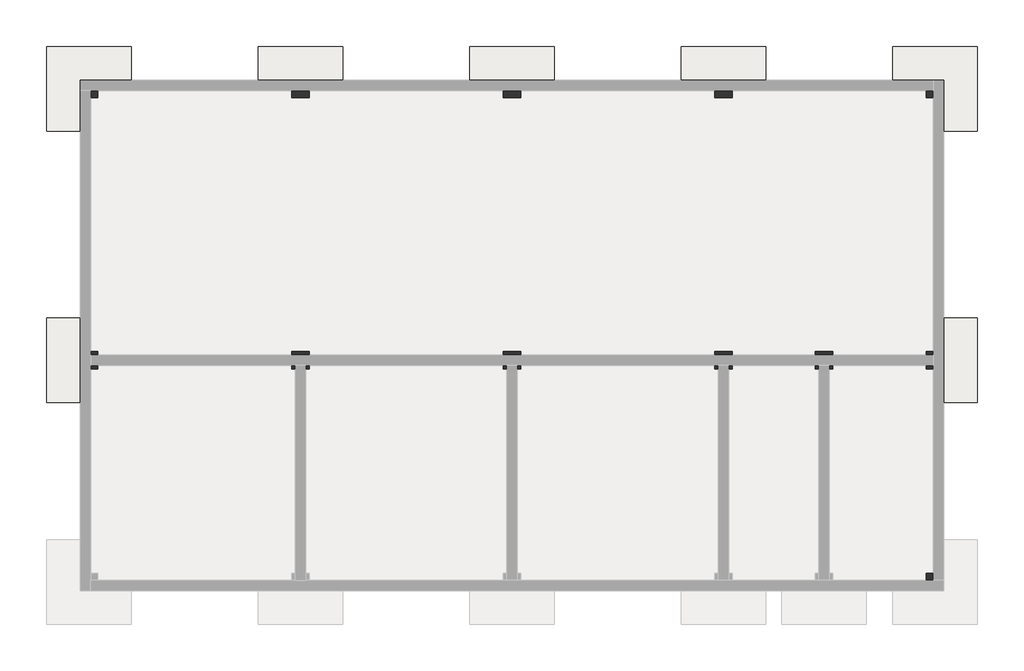
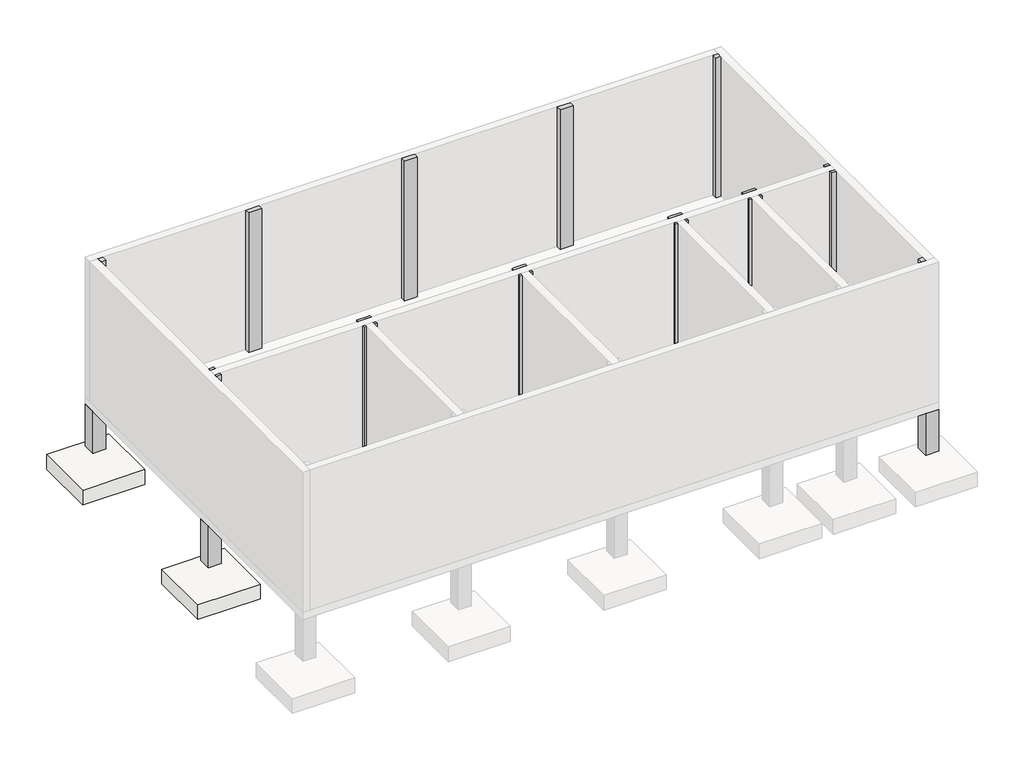
# One storey, part 2 of 2: 24 columns, 11 slabs.
"""IFC4 building model written with IfcOpenShell, lengths in millimetres."""

import ifcopenshell
import ifcopenshell.guid

model = None  # the IFC model being written
_history = None  # IfcOwnerHistory: only IFC2X3 demands one
_inside = {}  # id of a spatial element -> (the spatial element, [elements in it])
_under = {}  # id of a project, library or spatial element -> (it, [spatial elements below it])
_declared = {}  # id of a project -> (the project, [libraries it declares])
_typed = {}  # id of a type object -> (the type object, [elements of that type])
_made_of = {}  # id of a material, layer set ... -> (it, [elements and type objects made of it])


def new_model(schema):
    """Start an empty IFC model of exactly this schema.

    Asked for "IFC4X3", IfcOpenShell would pick the latest addendum, in which some entities
    have other attributes; the version numbers below select the first issue.
    IFC2X3 requires an IfcOwnerHistory on every rooted entity: one is made here for all.
    """
    global model, _history
    if schema == "IFC4X3":
        model = ifcopenshell.file(schema_version=(4, 3, 0, 0))
    else:
        model = ifcopenshell.file(schema=schema)
    _inside.clear()
    _under.clear()
    _declared.clear()
    _typed.clear()
    _made_of.clear()
    _history = None
    if model.schema == "IFC2X3":
        org = make("IfcOrganization", Name="unknown")
        user = make(
            "IfcPersonAndOrganization",
            ThePerson=make("IfcPerson", FamilyName="unknown"),
            TheOrganization=org,
        )
        app = make(
            "IfcApplication",
            ApplicationDeveloper=org,
            Version="unknown",
            ApplicationFullName="unknown",
            ApplicationIdentifier="unknown",
        )
        _history = make(
            "IfcOwnerHistory",
            OwningUser=user,
            OwningApplication=app,
            ChangeAction="ADDED",
            CreationDate=0,
        )
    return model


def make(cls, **values):
    """One entity of the class cls with the attributes given. An attribute that is None is left unset."""
    return model.create_entity(
        cls, **{name: value for name, value in values.items() if value is not None}
    )


def rooted(cls, **values):
    """An entity with a GlobalId (a new one), such as an element, a storey or a relation."""
    return make(cls, GlobalId=ifcopenshell.guid.new(), OwnerHistory=_history, **values)


def si_unit(unit_type, name, prefix=None):
    """IfcSIUnit, for example si_unit("LENGTHUNIT", "METRE", prefix="MILLI")."""
    return make("IfcSIUnit", UnitType=unit_type, Prefix=prefix, Name=name)


def assignment(units):
    """IfcUnitAssignment: the units of a project."""
    return None if units is None else make("IfcUnitAssignment", Units=units)


def point(xyz):
    """IfcCartesianPoint."""
    return None if xyz is None else make("IfcCartesianPoint", Coordinates=xyz)


def direction(xyz):
    """IfcDirection."""
    return None if xyz is None else make("IfcDirection", DirectionRatios=xyz)


def frame(location, z_axis=None, x_axis=None):
    """IfcAxis2Placement3D, a coordinate frame: its origin and axes. An axis left out is left unset."""
    return make(
        "IfcAxis2Placement3D",
        Location=point(location),
        Axis=direction(z_axis),
        RefDirection=direction(x_axis),
    )


def origin():
    """The frame at (0, 0, 0) with its axes left unset."""
    return frame((0.0, 0.0, 0.0))


def place(relative_to, where):
    """IfcLocalPlacement: puts the frame where relative to a parent placement (None: the world)."""
    return make(
        "IfcLocalPlacement", PlacementRelTo=relative_to, RelativePlacement=where
    )


def context(
    kind, dimensions, precision=None, world=None, true_north=None, identifier=None
):
    """IfcGeometricRepresentationContext, for example the 3D "Model" context."""
    return make(
        "IfcGeometricRepresentationContext",
        ContextIdentifier=identifier,
        ContextType=kind,
        CoordinateSpaceDimension=dimensions,
        Precision=precision,
        WorldCoordinateSystem=world,
        TrueNorth=true_north,
    )


def project(units=None, contexts=None):
    """IfcProject with its units and contexts."""
    return rooted(
        "IfcProject",
        Name="project",
        RepresentationContexts=contexts,
        UnitsInContext=assignment(units),
    )


def spatial(cls, under=None, at=None, **own):
    """A site, building, storey or space (cls), placed at a placement, below another one or the project."""
    s = rooted(cls, ObjectPlacement=at, **own)
    if under is not None:
        _under.setdefault(under.id(), (under, []))[1].append(s)
    return s


def polyline(points):
    """IfcPolyline through the points."""
    return make("IfcPolyline", Points=[point(p) for p in points])


def outline(outer, holes=None, kind="AREA"):
    """IfcArbitraryClosedProfileDef: a profile drawn as a closed curve; with holes, ...WithVoids."""
    if holes is None:
        return make("IfcArbitraryClosedProfileDef", ProfileType=kind, OuterCurve=outer)
    return make(
        "IfcArbitraryProfileDefWithVoids",
        ProfileType=kind,
        OuterCurve=outer,
        InnerCurves=holes,
    )


def extrude(swept, where, along, depth):
    """IfcExtrudedAreaSolid: the profile swept, set in the frame where, extruded along a direction by depth."""
    return make(
        "IfcExtrudedAreaSolid",
        SweptArea=swept,
        Position=where,
        ExtrudedDirection=direction(along),
        Depth=depth,
    )


def faces_of(points, faces, orient=None, outer=None):
    """IfcFace entities. A face is a list of loops; a loop is a list of indices into points, from 0.

    orient and outer hold one flag for each loop. By default every Orientation is true, the
    first loop of a face is its IfcFaceOuterBound and the others are IfcFaceBound.
    """
    made = []
    for i, loops in enumerate(faces):
        bounds = []
        for j, loop in enumerate(loops):
            is_outer = j == 0 if outer is None else outer[i][j]
            bounds.append(
                make(
                    "IfcFaceOuterBound" if is_outer else "IfcFaceBound",
                    Bound=make("IfcPolyLoop", Polygon=[points[k] for k in loop]),
                    Orientation=True if orient is None else orient[i][j],
                )
            )
        made.append(make("IfcFace", Bounds=bounds))
    return made


def faceted_brep(points, faces, orient=None, outer=None, voids=None):
    """IfcFacetedBrep: a solid bounded by flat faces; with voids (closed shells), ...WithVoids."""
    shared = [point(p) for p in points]
    hull = make("IfcClosedShell", CfsFaces=faces_of(shared, faces, orient, outer))
    if voids is None:
        return make("IfcFacetedBrep", Outer=hull)
    return make(
        "IfcFacetedBrepWithVoids",
        Outer=hull,
        Voids=[
            make(cls, CfsFaces=faces_of(shared, fs, o, b)) for cls, fs, o, b in voids
        ],
    )


def shape(context_of_items, identifier, shape_type, items):
    """IfcShapeRepresentation: the items that make up one representation, for example the "Body"."""
    return make(
        "IfcShapeRepresentation",
        ContextOfItems=context_of_items,
        RepresentationIdentifier=identifier,
        RepresentationType=shape_type,
        Items=items,
    )


def source(mapping_origin, context_of_items, identifier, shape_type, items):
    """IfcRepresentationMap: a shape defined once, which mapped items show again and again."""
    return make(
        "IfcRepresentationMap",
        MappingOrigin=mapping_origin,
        MappedRepresentation=shape(context_of_items, identifier, shape_type, items),
    )


def transform(
    local_origin,
    x_axis=None,
    y_axis=None,
    z_axis=None,
    scale=None,
    scale2=None,
    scale3=None,
    uniform=True,
):
    """IfcCartesianTransformationOperator3D, or its non-uniform kind. x_axis, y_axis, z_axis: its Axis1, 2, 3."""
    if uniform:
        return make(
            "IfcCartesianTransformationOperator3D",
            Axis1=direction(x_axis),
            Axis2=direction(y_axis),
            LocalOrigin=point(local_origin),
            Scale=scale,
            Axis3=direction(z_axis),
        )
    return make(
        "IfcCartesianTransformationOperator3DnonUniform",
        Axis1=direction(x_axis),
        Axis2=direction(y_axis),
        LocalOrigin=point(local_origin),
        Scale=scale,
        Axis3=direction(z_axis),
        Scale2=scale2,
        Scale3=scale3,
    )


def mapped(mapping_source, mapping_target):
    """IfcMappedItem: shows the shape of a source again, moved by a transform."""
    return make(
        "IfcMappedItem", MappingSource=mapping_source, MappingTarget=mapping_target
    )


def made_of(thing, what):
    """Note that an element or type object is made of a material, layer set ...; save() writes the relation."""
    if what is not None:
        _made_of.setdefault(what.id(), (what, []))[1].append(thing)
    return thing


def element(
    cls,
    number,
    at=None,
    inside=None,
    cuts=None,
    type_object=None,
    material=None,
    context=None,
    identifier="Body",
    shape_type=None,
    held_by="IfcProductDefinitionShape",
    body=None,
    shapes=None,
    **own,
):
    """One element of the class cls, such as IfcWall. Its Tag is "e" and its number.

    at: its placement. inside: the storey or other place that contains it. cuts: it is an
    opening in that element (IfcRelVoidsElement). A single representation is given by context,
    identifier, shape_type and body (its items); several are given by shapes. held_by: the class
    of the entity that holds the representations. save() writes the other relations.
    """
    e = rooted(cls, Tag="e%d" % number, ObjectPlacement=at, **own)
    if body is not None:
        shapes = [shape(context, identifier, shape_type, body)]
    if shapes is not None:
        e.Representation = make(held_by, Representations=shapes)
    if inside is not None:
        _inside.setdefault(inside.id(), (inside, []))[1].append(e)
    if cuts is not None:
        rooted(
            "IfcRelVoidsElement", RelatingBuildingElement=cuts, RelatedOpeningElement=e
        )
    if type_object is not None:
        _typed.setdefault(type_object.id(), (type_object, []))[1].append(e)
    return made_of(e, material)


def aggregate(whole, parts):
    """IfcRelAggregates: a whole, such as a stair, and the parts it consists of."""
    return rooted("IfcRelAggregates", RelatingObject=whole, RelatedObjects=parts)


def save(model, path):
    """Write the relations noted so far, then the file.

    IfcRelAggregates (storeys below a building ...), IfcRelContainedInSpatialStructure (elements
    in a storey), IfcRelDefinesByType, IfcRelAssociatesMaterial and IfcRelDeclares: one each for
    every whole, place, type object, material and project.
    """
    for whole, parts in _under.values():
        aggregate(whole, parts)
    for where, things in _inside.values():
        rooted(
            "IfcRelContainedInSpatialStructure",
            RelatedElements=things,
            RelatingStructure=where,
        )
    for kind, things in _typed.values():
        rooted("IfcRelDefinesByType", RelatedObjects=things, RelatingType=kind)
    for what, things in _made_of.values():
        rooted("IfcRelAssociatesMaterial", RelatedObjects=things, RelatingMaterial=what)
    for by, libraries in _declared.values():
        rooted("IfcRelDeclares", RelatingContext=by, RelatedDefinitions=libraries)
    model.write(path)


def foundation_rectangular_non_pile_2400_x_2400_x_600mm_9fdc1d6b(model_context):
    return source(origin(), model_context, "Body", "SweptSolid", [
        extrude(outline(polyline([(1200.0, 1200.0), (1200.0, -1200.0), (-1200.0, -1200.0), (-1200.0, 1200.0), (1200.0, 1200.0)])), frame((0.0, 0.0, -600.0), z_axis=(0.0, 0.0, 1.0), x_axis=(1.0, 0.0, 0.0)), (0.0, 0.0, 1.0), 600.0),
    ])


model = new_model("IFC4")

# Units and contexts
model_context = context("Model", 3, world=origin())
ifc_project = project(units=[si_unit("LENGTHUNIT", "METRE", prefix="MILLI")], contexts=[model_context])

# Site, building, storey
site = spatial("IfcSite", under=ifc_project)
building = spatial("IfcBuilding", under=site)
storey = spatial("IfcBuildingStorey", under=building, Name="1st FL GL+200", Elevation=0.0)

# Columns
placement = place(None, origin())
element("IfcColumn", 1, ObjectType="RC_Column_Rectangular : 500 x 500mm", at=placement, inside=storey, context=model_context, shape_type="SweptSolid", body=[
    extrude(outline(polyline([(-18445.7273237, 9685.9763125), (-18445.7273237, 9185.9763125), (-18945.7273237, 9185.9763125), (-18945.7273237, 9685.9763125), (-18445.7273237, 9685.9763125)])), frame((0.0, 0.0, -2000.0), z_axis=(0.0, 0.0, 1.0), x_axis=(1.0, 0.0, 0.0)), (0.0, 0.0, 1.0), 1700.0),
])
element("IfcColumn", 2, ObjectType="RC_Column_Rectangular : 500 x 500mm", at=placement, inside=storey, context=model_context, shape_type="SweptSolid", body=[
    extrude(outline(polyline([(-18445.7273237, 1985.9763125), (-18445.7273237, 1485.9763125), (-18945.7273237, 1485.9763125), (-18945.7273237, 1985.9763125), (-18445.7273237, 1985.9763125)])), frame((0.0, 0.0, -2000.0), z_axis=(0.0, 0.0, 1.0), x_axis=(1.0, 0.0, 0.0)), (0.0, 0.0, 1.0), 1700.0),
])
element("IfcColumn", 3, ObjectType="RC_Column_Rectangular : 500 x 500mm", at=placement, inside=storey, context=model_context, shape_type="SweptSolid", body=[
    extrude(outline(polyline([(-12445.7273237, 9685.9763125), (-12445.7273237, 9185.9763125), (-12945.7273237, 9185.9763125), (-12945.7273237, 9685.9763125), (-12445.7273237, 9685.9763125)])), frame((0.0, 0.0, -2000.0), z_axis=(0.0, 0.0, 1.0), x_axis=(1.0, 0.0, 0.0)), (0.0, 0.0, 1.0), 1700.0),
])
element("IfcColumn", 4, ObjectType="RC_Column_Rectangular : 500 x 500mm", at=placement, inside=storey, context=model_context, shape_type="SweptSolid", body=[
    extrude(outline(polyline([(-12445.7273237, 1985.9763125), (-12445.7273237, 1485.9763125), (-12945.7273237, 1485.9763125), (-12945.7273237, 1985.9763125), (-12445.7273237, 1985.9763125)])), frame((0.0, 0.0, -2000.0), z_axis=(0.0, 0.0, 1.0), x_axis=(1.0, 0.0, 0.0)), (0.0, 0.0, 1.0), 1700.0),
])
element("IfcColumn", 5, ObjectType="RC_Column_Rectangular : 500 x 500mm", at=placement, inside=storey, context=model_context, shape_type="SweptSolid", body=[
    extrude(outline(polyline([(-6445.7273237, 9685.9763125), (-6445.7273237, 9185.9763125), (-6945.7273237, 9185.9763125), (-6945.7273237, 9685.9763125), (-6445.7273237, 9685.9763125)])), frame((0.0, 0.0, -2000.0), z_axis=(0.0, 0.0, 1.0), x_axis=(1.0, 0.0, 0.0)), (0.0, 0.0, 1.0), 1700.0),
])
element("IfcColumn", 6, ObjectType="RC_Column_Rectangular : 500 x 500mm", at=placement, inside=storey, context=model_context, shape_type="SweptSolid", body=[
    extrude(outline(polyline([(-6445.7273237, 1985.9763125), (-6445.7273237, 1485.9763125), (-6945.7273237, 1485.9763125), (-6945.7273237, 1985.9763125), (-6445.7273237, 1985.9763125)])), frame((0.0, 0.0, -2000.0), z_axis=(0.0, 0.0, 1.0), x_axis=(1.0, 0.0, 0.0)), (0.0, 0.0, 1.0), 1700.0),
])
element("IfcColumn", 7, ObjectType="RC_Column_Rectangular : 500 x 500mm", at=placement, inside=storey, context=model_context, shape_type="SweptSolid", body=[
    extrude(outline(polyline([(-445.7273237, 9685.9763125), (-445.7273237, 9185.9763125), (-945.7273237, 9185.9763125), (-945.7273237, 9685.9763125), (-445.7273237, 9685.9763125)])), frame((0.0, 0.0, -2000.0), z_axis=(0.0, 0.0, 1.0), x_axis=(1.0, 0.0, 0.0)), (0.0, 0.0, 1.0), 1700.0),
])
element("IfcColumn", 8, ObjectType="RC_Column_Rectangular : 500 x 500mm", at=placement, inside=storey, context=model_context, shape_type="SweptSolid", body=[
    extrude(outline(polyline([(-445.7273237, 1985.9763125), (-445.7273237, 1485.9763125), (-945.7273237, 1485.9763125), (-945.7273237, 1985.9763125), (-445.7273237, 1985.9763125)])), frame((0.0, 0.0, -2000.0), z_axis=(0.0, 0.0, 1.0), x_axis=(1.0, 0.0, 0.0)), (0.0, 0.0, 1.0), 1700.0),
])
element("IfcColumn", 9, ObjectType="RC_Column_Rectangular : 500 x 500mm", at=placement, inside=storey, context=model_context, shape_type="SweptSolid", body=[
    extrude(outline(polyline([(5554.2726763, 9685.9763125), (5554.2726763, 9185.9763125), (5054.2726763, 9185.9763125), (5054.2726763, 9685.9763125), (5554.2726763, 9685.9763125)])), frame((0.0, 0.0, -2000.0), z_axis=(0.0, 0.0, 1.0), x_axis=(1.0, 0.0, 0.0)), (0.0, 0.0, 1.0), 1700.0),
])
element("IfcColumn", 10, ObjectType="RC_Column_Rectangular : 500 x 500mm", at=placement, inside=storey, context=model_context, shape_type="SweptSolid", body=[
    extrude(outline(polyline([(5554.2726763, 1985.9763125), (5554.2726763, 1485.9763125), (5054.2726763, 1485.9763125), (5054.2726763, 1985.9763125), (5554.2726763, 1985.9763125)])), frame((0.0, 0.0, -2000.0), z_axis=(0.0, 0.0, 1.0), x_axis=(1.0, 0.0, 0.0)), (0.0, 0.0, 1.0), 1700.0),
])
element("IfcColumn", 11, ObjectType="RC_Column_Rectangular : 500 x 500mm", at=placement, inside=storey, context=model_context, shape_type="SweptSolid", body=[
    extrude(outline(polyline([(5554.2726763, -4314.0236875), (5554.2726763, -4814.0236875), (5054.2726763, -4814.0236875), (5054.2726763, -4314.0236875), (5554.2726763, -4314.0236875)])), frame((0.0, 0.0, -2000.0), z_axis=(0.0, 0.0, 1.0), x_axis=(1.0, 0.0, 0.0)), (0.0, 0.0, 1.0), 1700.0),
])
element("IfcColumn", 12, ObjectType="RC_Column_Rectangular : 500 x 500mm", at=placement, inside=storey, context=model_context, shape_type="SweptSolid", body=[
    extrude(outline(polyline([(2404.2726763, 1985.9763125), (2404.2726763, 1485.9763125), (1904.2726763, 1485.9763125), (1904.2726763, 1985.9763125), (2404.2726763, 1985.9763125)])), frame((0.0, 0.0, -2000.0), z_axis=(0.0, 0.0, 1.0), x_axis=(1.0, 0.0, 0.0)), (0.0, 0.0, 1.0), 1700.0),
])
element("IfcColumn", 13, ObjectType="RC_Column_Rectangular : 500 x 500mm", at=placement, inside=storey, context=model_context, shape_type="Brep", body=[
    faceted_brep([(-18445.7273237, 9385.9763125, 0.0), (-18445.7273237, 9185.9763125, 0.0), (-18645.7273237, 9185.9763125, 0.0), (-18645.7273237, 9385.9763125, 0.0), (-18445.7273237, 9185.9763125, 5700.0), (-18595.7273237, 9185.9763125, 5700.0), (-18645.7273237, 9185.9763125, 5700.0), (-18645.7273237, 9185.9763125, 5300.0), (-18445.7273237, 9385.9763125, 5700.0), (-18645.7273237, 9385.9763125, 5700.0)], [[[0, 1, 2, 3]], [[1, 4, 5, 6, 7, 2]], [[4, 1, 0, 8]], [[4, 8, 9, 6, 5]], [[8, 0, 3, 9]], [[3, 2, 7, 6, 9]]]),
])
element("IfcColumn", 14, ObjectType="RC_Column_Rectangular : 500 x 500mm", at=placement, inside=storey, context=model_context, shape_type="Brep", body=[
    faceted_brep([(-18645.7273237, 1985.9763125, 0.0), (-18445.7273237, 1985.9763125, 0.0), (-18445.7273237, 1885.9763125, 0.0), (-18645.7273237, 1885.9763125, 0.0), (-18445.7273237, 1985.9763125, 5700.0), (-18645.7273237, 1985.9763125, 5300.0), (-18645.7273237, 1985.9763125, 5700.0), (-18595.7273237, 1985.9763125, 5700.0), (-18445.7273237, 1910.9763125, 5700.0), (-18445.7273237, 1885.9763125, 5700.0), (-18445.7273237, 1885.9763125, 5300.0), (-18645.7273237, 1885.9763125, 5700.0)], [[[0, 1, 2, 3]], [[4, 1, 0, 5, 6, 7]], [[1, 4, 8, 9, 10, 2]], [[3, 2, 10, 9, 11]], [[4, 7, 6, 11, 9, 8]], [[6, 5, 0, 3, 11]]]),
    faceted_brep([(-18445.7273237, 1485.9763125, 0.0), (-18445.7273237, 1485.9763125, 5700.0), (-18595.7273237, 1485.9763125, 5700.0), (-18645.7273237, 1485.9763125, 5700.0), (-18645.7273237, 1485.9763125, 5300.0), (-18645.7273237, 1485.9763125, 0.0), (-18445.7273237, 1560.9763125, 5700.0), (-18445.7273237, 1585.9763125, 5700.0), (-18645.7273237, 1585.9763125, 5700.0), (-18645.7273237, 1585.9763125, 0.0), (-18445.7273237, 1585.9763125, 0.0), (-18445.7273237, 1585.9763125, 5300.0)], [[[0, 1, 2, 3, 4, 5]], [[3, 2, 1, 6, 7, 8]], [[5, 4, 3, 8, 9]], [[10, 9, 8, 7, 11]], [[0, 5, 9, 10]], [[1, 0, 10, 11, 7, 6]]]),
])
element("IfcColumn", 15, ObjectType="RC_Column_Rectangular : 500 x 500mm", at=placement, inside=storey, context=model_context, shape_type="Brep", body=[
    faceted_brep([(-12445.7273237, 9185.9763125, 0.0), (-12945.7273237, 9185.9763125, 0.0), (-12945.7273237, 9385.9763125, 0.0), (-12445.7273237, 9385.9763125, 0.0), (-12945.7273237, 9185.9763125, 5700.0), (-12945.7273237, 9335.9763125, 5700.0), (-12945.7273237, 9385.9763125, 5700.0), (-12945.7273237, 9385.9763125, 5300.0), (-12445.7273237, 9185.9763125, 5700.0), (-12520.7273237, 9185.9763125, 5700.0), (-12870.7273237, 9185.9763125, 5700.0), (-12445.7273237, 9385.9763125, 5300.0), (-12445.7273237, 9385.9763125, 5700.0), (-12445.7273237, 9335.9763125, 5700.0)], [[[0, 1, 2, 3]], [[1, 4, 5, 6, 7, 2]], [[1, 0, 8, 9, 10, 4]], [[8, 0, 3, 11, 12, 13]], [[4, 10, 9, 8, 13, 12, 6, 5]], [[3, 2, 7, 6, 12, 11]]]),
])
element("IfcColumn", 16, ObjectType="RC_Column_Rectangular : 500 x 500mm", at=placement, inside=storey, context=model_context, shape_type="Brep", body=[
    faceted_brep([(-12945.7273237, 1985.9763125, 0.0), (-12445.7273237, 1985.9763125, 0.0), (-12445.7273237, 1885.9763125, 0.0), (-12945.7273237, 1885.9763125, 0.0), (-12945.7273237, 1985.9763125, 5700.0), (-12870.7273237, 1985.9763125, 5700.0), (-12520.7273237, 1985.9763125, 5700.0), (-12445.7273237, 1985.9763125, 5700.0), (-12945.7273237, 1885.9763125, 5300.0), (-12945.7273237, 1885.9763125, 5700.0), (-12945.7273237, 1910.9763125, 5700.0), (-12445.7273237, 1910.9763125, 5700.0), (-12445.7273237, 1885.9763125, 5700.0), (-12445.7273237, 1885.9763125, 5300.0)], [[[0, 1, 2, 3]], [[1, 0, 4, 5, 6, 7]], [[4, 0, 3, 8, 9, 10]], [[1, 7, 11, 12, 13, 2]], [[3, 2, 13, 12, 9, 8]], [[7, 6, 5, 4, 10, 9, 12, 11]]]),
    faceted_brep([(-12945.7273237, 1485.9763125, 5700.0), (-12945.7273237, 1485.9763125, 0.0), (-12845.7273237, 1485.9763125, 0.0), (-12845.7273237, 1485.9763125, 5300.0), (-12845.7273237, 1485.9763125, 5700.0), (-12870.7273237, 1485.9763125, 5700.0), (-12945.7273237, 1585.9763125, 0.0), (-12945.7273237, 1585.9763125, 5300.0), (-12945.7273237, 1585.9763125, 5700.0), (-12845.7273237, 1585.9763125, 5700.0), (-12845.7273237, 1585.9763125, 0.0), (-12945.7273237, 1560.9763125, 5700.0)], [[[0, 1, 2, 3, 4, 5]], [[6, 7, 8, 9, 10]], [[1, 6, 10, 2]], [[1, 0, 11, 8, 7, 6]], [[4, 3, 2, 10, 9]], [[8, 11, 0, 5, 4, 9]]]),
    faceted_brep([(-12445.7273237, 1485.9763125, 5700.0), (-12445.7273237, 1560.9763125, 5700.0), (-12445.7273237, 1585.9763125, 5700.0), (-12545.7273237, 1585.9763125, 5700.0), (-12545.7273237, 1485.9763125, 5700.0), (-12520.7273237, 1485.9763125, 5700.0), (-12445.7273237, 1485.9763125, 0.0), (-12445.7273237, 1585.9763125, 0.0), (-12445.7273237, 1585.9763125, 5300.0), (-12545.7273237, 1485.9763125, 0.0), (-12545.7273237, 1485.9763125, 5300.0), (-12545.7273237, 1585.9763125, 0.0)], [[[0, 1, 2, 3, 4, 5]], [[0, 6, 7, 8, 2, 1]], [[9, 10, 4, 3, 11]], [[6, 0, 5, 4, 10, 9]], [[2, 8, 7, 11, 3]], [[7, 6, 9, 11]]]),
])
element("IfcColumn", 17, ObjectType="RC_Column_Rectangular : 500 x 500mm", at=placement, inside=storey, context=model_context, shape_type="Brep", body=[
    faceted_brep([(-6445.7273237, 9185.9763125, 0.0), (-6945.7273237, 9185.9763125, 0.0), (-6945.7273237, 9385.9763125, 0.0), (-6445.7273237, 9385.9763125, 0.0), (-6945.7273237, 9185.9763125, 5700.0), (-6945.7273237, 9335.9763125, 5700.0), (-6945.7273237, 9385.9763125, 5700.0), (-6945.7273237, 9385.9763125, 5300.0), (-6445.7273237, 9185.9763125, 5700.0), (-6520.7273237, 9185.9763125, 5700.0), (-6870.7273237, 9185.9763125, 5700.0), (-6445.7273237, 9385.9763125, 5300.0), (-6445.7273237, 9385.9763125, 5700.0), (-6445.7273237, 9335.9763125, 5700.0)], [[[0, 1, 2, 3]], [[1, 4, 5, 6, 7, 2]], [[1, 0, 8, 9, 10, 4]], [[8, 0, 3, 11, 12, 13]], [[4, 10, 9, 8, 13, 12, 6, 5]], [[3, 2, 7, 6, 12, 11]]]),
])
element("IfcColumn", 18, ObjectType="RC_Column_Rectangular : 500 x 500mm", at=placement, inside=storey, context=model_context, shape_type="Brep", body=[
    faceted_brep([(-6945.7273237, 1985.9763125, 0.0), (-6445.7273237, 1985.9763125, 0.0), (-6445.7273237, 1885.9763125, 0.0), (-6945.7273237, 1885.9763125, 0.0), (-6945.7273237, 1985.9763125, 5700.0), (-6870.7273237, 1985.9763125, 5700.0), (-6520.7273237, 1985.9763125, 5700.0), (-6445.7273237, 1985.9763125, 5700.0), (-6945.7273237, 1885.9763125, 5300.0), (-6945.7273237, 1885.9763125, 5700.0), (-6945.7273237, 1910.9763125, 5700.0), (-6445.7273237, 1910.9763125, 5700.0), (-6445.7273237, 1885.9763125, 5700.0), (-6445.7273237, 1885.9763125, 5300.0)], [[[0, 1, 2, 3]], [[1, 0, 4, 5, 6, 7]], [[4, 0, 3, 8, 9, 10]], [[1, 7, 11, 12, 13, 2]], [[3, 2, 13, 12, 9, 8]], [[7, 6, 5, 4, 10, 9, 12, 11]]]),
    faceted_brep([(-6945.7273237, 1485.9763125, 5700.0), (-6945.7273237, 1485.9763125, 0.0), (-6845.7273237, 1485.9763125, 0.0), (-6845.7273237, 1485.9763125, 5300.0), (-6845.7273237, 1485.9763125, 5700.0), (-6870.7273237, 1485.9763125, 5700.0), (-6945.7273237, 1585.9763125, 0.0), (-6945.7273237, 1585.9763125, 5300.0), (-6945.7273237, 1585.9763125, 5700.0), (-6845.7273237, 1585.9763125, 5700.0), (-6845.7273237, 1585.9763125, 0.0), (-6945.7273237, 1560.9763125, 5700.0)], [[[0, 1, 2, 3, 4, 5]], [[6, 7, 8, 9, 10]], [[1, 6, 10, 2]], [[1, 0, 11, 8, 7, 6]], [[4, 3, 2, 10, 9]], [[8, 11, 0, 5, 4, 9]]]),
    faceted_brep([(-6445.7273237, 1485.9763125, 5700.0), (-6445.7273237, 1560.9763125, 5700.0), (-6445.7273237, 1585.9763125, 5700.0), (-6545.7273237, 1585.9763125, 5700.0), (-6545.7273237, 1485.9763125, 5700.0), (-6520.7273237, 1485.9763125, 5700.0), (-6445.7273237, 1485.9763125, 0.0), (-6445.7273237, 1585.9763125, 0.0), (-6445.7273237, 1585.9763125, 5300.0), (-6545.7273237, 1485.9763125, 0.0), (-6545.7273237, 1485.9763125, 5300.0), (-6545.7273237, 1585.9763125, 0.0)], [[[0, 1, 2, 3, 4, 5]], [[0, 6, 7, 8, 2, 1]], [[9, 10, 4, 3, 11]], [[6, 0, 5, 4, 10, 9]], [[2, 8, 7, 11, 3]], [[7, 6, 9, 11]]]),
])
element("IfcColumn", 19, ObjectType="RC_Column_Rectangular : 500 x 500mm", at=placement, inside=storey, context=model_context, shape_type="Brep", body=[
    faceted_brep([(-445.7273237, 9185.9763125, 0.0), (-945.7273237, 9185.9763125, 0.0), (-945.7273237, 9385.9763125, 0.0), (-445.7273237, 9385.9763125, 0.0), (-945.7273237, 9185.9763125, 5700.0), (-945.7273237, 9335.9763125, 5700.0), (-945.7273237, 9385.9763125, 5700.0), (-945.7273237, 9385.9763125, 5300.0), (-445.7273237, 9185.9763125, 5700.0), (-520.7273237, 9185.9763125, 5700.0), (-870.7273237, 9185.9763125, 5700.0), (-445.7273237, 9385.9763125, 5700.0)], [[[0, 1, 2, 3]], [[1, 4, 5, 6, 7, 2]], [[1, 0, 8, 9, 10, 4]], [[8, 0, 3, 11]], [[4, 10, 9, 8, 11, 6, 5]], [[3, 2, 7, 6, 11]]]),
])
element("IfcColumn", 20, ObjectType="RC_Column_Rectangular : 500 x 500mm", at=placement, inside=storey, context=model_context, shape_type="Brep", body=[
    faceted_brep([(-945.7273237, 1985.9763125, 0.0), (-445.7273237, 1985.9763125, 0.0), (-445.7273237, 1885.9763125, 0.0), (-945.7273237, 1885.9763125, 0.0), (-945.7273237, 1985.9763125, 5700.0), (-870.7273237, 1985.9763125, 5700.0), (-520.7273237, 1985.9763125, 5700.0), (-445.7273237, 1985.9763125, 5700.0), (-945.7273237, 1885.9763125, 5300.0), (-945.7273237, 1885.9763125, 5700.0), (-945.7273237, 1910.9763125, 5700.0), (-445.7273237, 1910.9763125, 5700.0), (-445.7273237, 1885.9763125, 5700.0), (-445.7273237, 1885.9763125, 5300.0)], [[[0, 1, 2, 3]], [[1, 0, 4, 5, 6, 7]], [[4, 0, 3, 8, 9, 10]], [[1, 7, 11, 12, 13, 2]], [[3, 2, 13, 12, 9, 8]], [[7, 6, 5, 4, 10, 9, 12, 11]]]),
    faceted_brep([(-945.7273237, 1485.9763125, 5700.0), (-945.7273237, 1485.9763125, 0.0), (-845.7273237, 1485.9763125, 0.0), (-845.7273237, 1485.9763125, 5300.0), (-845.7273237, 1485.9763125, 5700.0), (-870.7273237, 1485.9763125, 5700.0), (-945.7273237, 1585.9763125, 0.0), (-945.7273237, 1585.9763125, 5300.0), (-945.7273237, 1585.9763125, 5700.0), (-845.7273237, 1585.9763125, 5700.0), (-845.7273237, 1585.9763125, 0.0), (-945.7273237, 1560.9763125, 5700.0)], [[[0, 1, 2, 3, 4, 5]], [[6, 7, 8, 9, 10]], [[1, 6, 10, 2]], [[1, 0, 11, 8, 7, 6]], [[4, 3, 2, 10, 9]], [[8, 11, 0, 5, 4, 9]]]),
    faceted_brep([(-445.7273237, 1485.9763125, 5700.0), (-445.7273237, 1560.9763125, 5700.0), (-445.7273237, 1585.9763125, 5700.0), (-545.7273237, 1585.9763125, 5700.0), (-545.7273237, 1485.9763125, 5700.0), (-520.7273237, 1485.9763125, 5700.0), (-445.7273237, 1485.9763125, 0.0), (-445.7273237, 1585.9763125, 0.0), (-445.7273237, 1585.9763125, 5300.0), (-545.7273237, 1485.9763125, 0.0), (-545.7273237, 1485.9763125, 5300.0), (-545.7273237, 1585.9763125, 0.0)], [[[0, 1, 2, 3, 4, 5]], [[0, 6, 7, 8, 2, 1]], [[9, 10, 4, 3, 11]], [[6, 0, 5, 4, 10, 9]], [[2, 8, 7, 11, 3]], [[7, 6, 9, 11]]]),
])
element("IfcColumn", 21, ObjectType="RC_Column_Rectangular : 500 x 500mm", at=placement, inside=storey, context=model_context, shape_type="Brep", body=[
    faceted_brep([(5054.2726763, 9185.9763125, 0.0), (5054.2726763, 9385.9763125, 0.0), (5254.2726763, 9385.9763125, 0.0), (5254.2726763, 9185.9763125, 0.0), (5054.2726763, 9185.9763125, 5700.0), (5054.2726763, 9385.9763125, 5700.0), (5254.2726763, 9185.9763125, 5300.0), (5254.2726763, 9185.9763125, 5700.0), (5204.2726763, 9185.9763125, 5700.0), (5254.2726763, 9385.9763125, 5700.0)], [[[0, 1, 2, 3]], [[0, 4, 5, 1]], [[4, 0, 3, 6, 7, 8]], [[5, 4, 8, 7, 9]], [[2, 1, 5, 9]], [[3, 2, 9, 7, 6]]]),
])
element("IfcColumn", 22, ObjectType="RC_Column_Rectangular : 500 x 500mm", at=placement, inside=storey, context=model_context, shape_type="Brep", body=[
    faceted_brep([(5054.2726763, 1985.9763125, 0.0), (5254.2726763, 1985.9763125, 0.0), (5254.2726763, 1885.9763125, 0.0), (5054.2726763, 1885.9763125, 0.0), (5054.2726763, 1985.9763125, 5700.0), (5254.2726763, 1985.9763125, 5700.0), (5054.2726763, 1885.9763125, 5300.0), (5054.2726763, 1885.9763125, 5700.0), (5054.2726763, 1910.9763125, 5700.0), (5254.2726763, 1885.9763125, 5700.0)], [[[0, 1, 2, 3]], [[0, 4, 5, 1]], [[4, 0, 3, 6, 7, 8]], [[1, 5, 9, 2]], [[3, 2, 9, 7, 6]], [[5, 4, 8, 7, 9]]]),
    faceted_brep([(5054.2726763, 1485.9763125, 5700.0), (5054.2726763, 1485.9763125, 0.0), (5254.2726763, 1485.9763125, 0.0), (5254.2726763, 1485.9763125, 5300.0), (5254.2726763, 1485.9763125, 5700.0), (5204.2726763, 1485.9763125, 5700.0), (5254.2726763, 1585.9763125, 5700.0), (5054.2726763, 1585.9763125, 5700.0), (5054.2726763, 1560.9763125, 5700.0), (5254.2726763, 1585.9763125, 0.0), (5054.2726763, 1585.9763125, 0.0), (5054.2726763, 1585.9763125, 5300.0)], [[[0, 1, 2, 3, 4, 5]], [[0, 5, 4, 6, 7, 8]], [[9, 10, 11, 7, 6]], [[2, 1, 10, 9]], [[1, 0, 8, 7, 11, 10]], [[4, 3, 2, 9, 6]]]),
])
element("IfcColumn", 23, ObjectType="RC_Column_Rectangular : 500 x 500mm", at=placement, inside=storey, context=model_context, shape_type="Brep", body=[
    faceted_brep([(5054.2726763, -4514.0236875, 0.0), (5054.2726763, -4314.0236875, 0.0), (5254.2726763, -4314.0236875, 0.0), (5254.2726763, -4514.0236875, 0.0), (5054.2726763, -4314.0236875, 5700.0), (5204.2726763, -4314.0236875, 5700.0), (5254.2726763, -4314.0236875, 5700.0), (5254.2726763, -4314.0236875, 5300.0), (5054.2726763, -4514.0236875, 5700.0), (5254.2726763, -4514.0236875, 5700.0)], [[[0, 1, 2, 3]], [[1, 4, 5, 6, 7, 2]], [[4, 1, 0, 8]], [[4, 8, 9, 6, 5]], [[8, 0, 3, 9]], [[3, 2, 7, 6, 9]]]),
])
element("IfcColumn", 24, ObjectType="RC_Column_Rectangular : 500 x 500mm", at=placement, inside=storey, context=model_context, shape_type="Brep", body=[
    faceted_brep([(1904.2726763, 1985.9763125, 0.0), (2404.2726763, 1985.9763125, 0.0), (2404.2726763, 1885.9763125, 0.0), (1904.2726763, 1885.9763125, 0.0), (1904.2726763, 1985.9763125, 5700.0), (2404.2726763, 1985.9763125, 5700.0), (1904.2726763, 1885.9763125, 5300.0), (1904.2726763, 1885.9763125, 5700.0), (1904.2726763, 1910.9763125, 5700.0), (2404.2726763, 1910.9763125, 5700.0), (2404.2726763, 1885.9763125, 5700.0), (2404.2726763, 1885.9763125, 5300.0)], [[[0, 1, 2, 3]], [[1, 0, 4, 5]], [[4, 0, 3, 6, 7, 8]], [[1, 5, 9, 10, 11, 2]], [[3, 2, 11, 10, 7, 6]], [[5, 4, 8, 7, 10, 9]]]),
    faceted_brep([(1904.2726763, 1485.9763125, 5700.0), (1904.2726763, 1485.9763125, 0.0), (2004.2726763, 1485.9763125, 0.0), (2004.2726763, 1485.9763125, 5300.0), (2004.2726763, 1485.9763125, 5700.0), (1979.2726763, 1485.9763125, 5700.0), (1904.2726763, 1585.9763125, 0.0), (1904.2726763, 1585.9763125, 5300.0), (1904.2726763, 1585.9763125, 5700.0), (2004.2726763, 1585.9763125, 5700.0), (2004.2726763, 1585.9763125, 0.0), (1904.2726763, 1560.9763125, 5700.0)], [[[0, 1, 2, 3, 4, 5]], [[6, 7, 8, 9, 10]], [[1, 6, 10, 2]], [[1, 0, 11, 8, 7, 6]], [[4, 3, 2, 10, 9]], [[8, 11, 0, 5, 4, 9]]]),
    faceted_brep([(2404.2726763, 1485.9763125, 5700.0), (2404.2726763, 1560.9763125, 5700.0), (2404.2726763, 1585.9763125, 5700.0), (2304.2726763, 1585.9763125, 5700.0), (2304.2726763, 1485.9763125, 5700.0), (2329.2726763, 1485.9763125, 5700.0), (2404.2726763, 1485.9763125, 0.0), (2404.2726763, 1585.9763125, 0.0), (2404.2726763, 1585.9763125, 5300.0), (2304.2726763, 1485.9763125, 0.0), (2304.2726763, 1485.9763125, 5300.0), (2304.2726763, 1585.9763125, 0.0)], [[[0, 1, 2, 3, 4, 5]], [[0, 6, 7, 8, 2, 1]], [[9, 10, 4, 3, 11]], [[6, 0, 5, 4, 10, 9]], [[2, 8, 7, 11, 3]], [[7, 6, 9, 11]]]),
])

# Slabs
foundation_rectangular_non_pile_2400_x_2400_x_600mm_shape = foundation_rectangular_non_pile_2400_x_2400_x_600mm_9fdc1d6b(model_context)
element("IfcSlab", 25, ObjectType="Foundation Rectangular(Non-Pile) : 2400 x 2400 x 600mm", at=placement, inside=storey, context=model_context, shape_type="MappedRepresentation", body=[
    mapped(foundation_rectangular_non_pile_2400_x_2400_x_600mm_shape, transform((-18695.7273237, 9435.9763125, -2600.0), x_axis=(1.0, 0.0, 0.0), y_axis=(0.0, 1.0, 0.0), z_axis=(0.0, 0.0, 1.0))),
])
element("IfcSlab", 26, ObjectType="Foundation Rectangular(Non-Pile) : 2400 x 2400 x 600mm", at=placement, inside=storey, context=model_context, shape_type="MappedRepresentation", body=[
    mapped(foundation_rectangular_non_pile_2400_x_2400_x_600mm_shape, transform((-18695.7273237, 1735.9763125, -2600.0), x_axis=(1.0, 0.0, 0.0), y_axis=(0.0, 1.0, 0.0), z_axis=(0.0, 0.0, 1.0))),
])
element("IfcSlab", 27, ObjectType="Foundation Rectangular(Non-Pile) : 2400 x 2400 x 600mm", at=placement, inside=storey, context=model_context, shape_type="MappedRepresentation", body=[
    mapped(foundation_rectangular_non_pile_2400_x_2400_x_600mm_shape, transform((-12695.7273237, 9435.9763125, -2600.0), x_axis=(1.0, 0.0, 0.0), y_axis=(0.0, 1.0, 0.0), z_axis=(0.0, 0.0, 1.0))),
])
element("IfcSlab", 28, ObjectType="Foundation Rectangular(Non-Pile) : 2400 x 2400 x 600mm", at=placement, inside=storey, context=model_context, shape_type="MappedRepresentation", body=[
    mapped(foundation_rectangular_non_pile_2400_x_2400_x_600mm_shape, transform((-12695.7273237, 1735.9763125, -2600.0), x_axis=(1.0, 0.0, 0.0), y_axis=(0.0, 1.0, 0.0), z_axis=(0.0, 0.0, 1.0))),
])
element("IfcSlab", 29, ObjectType="Foundation Rectangular(Non-Pile) : 2400 x 2400 x 600mm", at=placement, inside=storey, context=model_context, shape_type="MappedRepresentation", body=[
    mapped(foundation_rectangular_non_pile_2400_x_2400_x_600mm_shape, transform((-6695.7273237, 9435.9763125, -2600.0), x_axis=(1.0, 0.0, 0.0), y_axis=(0.0, 1.0, 0.0), z_axis=(0.0, 0.0, 1.0))),
])
element("IfcSlab", 30, ObjectType="Foundation Rectangular(Non-Pile) : 2400 x 2400 x 600mm", at=placement, inside=storey, context=model_context, shape_type="MappedRepresentation", body=[
    mapped(foundation_rectangular_non_pile_2400_x_2400_x_600mm_shape, transform((-6695.7273237, 1735.9763125, -2600.0), x_axis=(1.0, 0.0, 0.0), y_axis=(0.0, 1.0, 0.0), z_axis=(0.0, 0.0, 1.0))),
])
element("IfcSlab", 31, ObjectType="Foundation Rectangular(Non-Pile) : 2400 x 2400 x 600mm", at=placement, inside=storey, context=model_context, shape_type="MappedRepresentation", body=[
    mapped(foundation_rectangular_non_pile_2400_x_2400_x_600mm_shape, transform((-695.7273237, 9435.9763125, -2600.0), x_axis=(1.0, 0.0, 0.0), y_axis=(0.0, 1.0, 0.0), z_axis=(0.0, 0.0, 1.0))),
])
element("IfcSlab", 32, ObjectType="Foundation Rectangular(Non-Pile) : 2400 x 2400 x 600mm", at=placement, inside=storey, context=model_context, shape_type="MappedRepresentation", body=[
    mapped(foundation_rectangular_non_pile_2400_x_2400_x_600mm_shape, transform((-695.7273237, 1735.9763125, -2600.0), x_axis=(1.0, 0.0, 0.0), y_axis=(0.0, 1.0, 0.0), z_axis=(0.0, 0.0, 1.0))),
])
element("IfcSlab", 33, ObjectType="Foundation Rectangular(Non-Pile) : 2400 x 2400 x 600mm", at=placement, inside=storey, context=model_context, shape_type="MappedRepresentation", body=[
    mapped(foundation_rectangular_non_pile_2400_x_2400_x_600mm_shape, transform((5304.2726763, 9435.9763125, -2600.0), x_axis=(1.0, 0.0, 0.0), y_axis=(0.0, 1.0, 0.0), z_axis=(0.0, 0.0, 1.0))),
])
element("IfcSlab", 34, ObjectType="Foundation Rectangular(Non-Pile) : 2400 x 2400 x 600mm", at=placement, inside=storey, context=model_context, shape_type="MappedRepresentation", body=[
    mapped(foundation_rectangular_non_pile_2400_x_2400_x_600mm_shape, transform((5304.2726763, 1735.9763125, -2600.0), x_axis=(1.0, 0.0, 0.0), y_axis=(0.0, 1.0, 0.0), z_axis=(0.0, 0.0, 1.0))),
])
element("IfcSlab", 35, ObjectType="Foundation Rectangular(Non-Pile) : 2400 x 2400 x 600mm", at=placement, inside=storey, context=model_context, shape_type="MappedRepresentation", body=[
    mapped(foundation_rectangular_non_pile_2400_x_2400_x_600mm_shape, transform((2154.2726763, 1735.9763125, -2600.0), x_axis=(1.0, 0.0, 0.0), y_axis=(0.0, 1.0, 0.0), z_axis=(0.0, 0.0, 1.0))),
])

save(model, "model.ifc")

# Revit data of these elements
# Type "RC_Column_Rectangular : 500 x 500mm"
#   b = 500 mm
#   h = 500 mm
#   Structural Material [instance default] = 콘크리트, 현장타설 회색
# Type "Foundation Rectangular(Non-Pile) : 2400 x 2400 x 600mm"
#   Width = 2400 mm
#   Length = 2400 mm
#   Foundation Thickness = 600 mm
#   Structural Material [instance default] = 콘크리트 - 현장타설 콘크리트
#   Assembly Code = ""
# Elements 1, 2, 3, 4, 5, 6, 7, 8, 9, 10, 11, 12, 13, 14, 15, 16, 17, 18, 19, 20, 21, 22, 23, 24 (IfcColumn, "RC_Column_Rectangular : 500 x 500mm")
#   Structural Material = 콘크리트, 현장타설 회색
#   Phase Created = 신축
#   Materials on its faces: "콘크리트, 현장타설 회색"
# Elements 25, 26, 27, 28, 29, 30, 31, 32, 33, 34, 35 (IfcSlab, "Foundation Rectangular(Non-Pile) : 2400 x 2400 x 600mm")
#   Structural Material = 콘크리트 - 현장타설 콘크리트
#   Phase Created = 신축
#   Materials on its faces: "콘크리트 - 현장타설 콘크리트"
# Materials
#   "콘크리트, 현장타설 회색": class "콘크리트", colour RGB 192 192 192, transparency 0, Description = "현장타설 콘크리트", Cost = 0
#   "콘크리트 - 현장타설 콘크리트": class "콘크리트", colour RGB 192 192 192, transparency 0, Cost = 0
